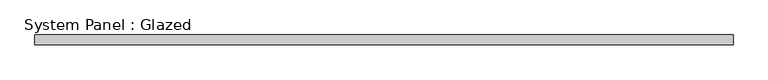
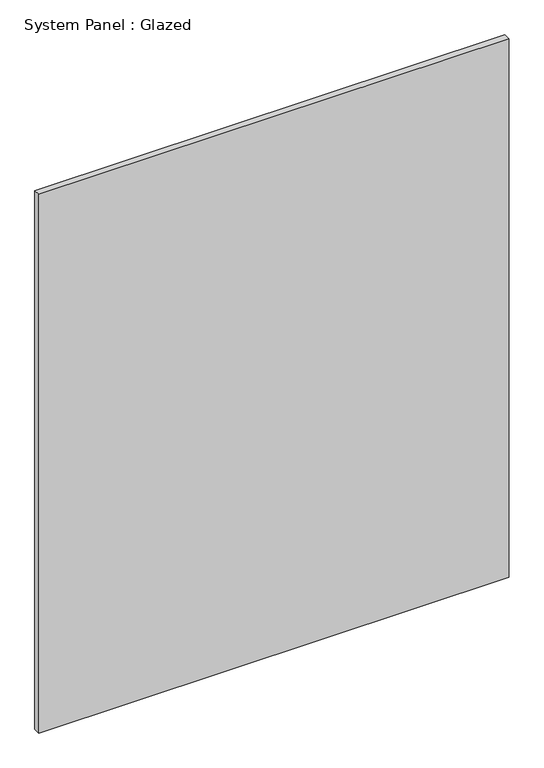
"""IFC4 building model written with IfcOpenShell, lengths in millimetres: plate geometry, System Panel : Glazed."""

from ifc_helpers import new_model, si_unit, origin, origin_with_axes, place, context, project, spatial, polyline, outline, extrude, source, transform, mapped, element, save


def system_panel_glazed_53184239(model_context):
    return source(origin(), model_context, "Body", "SweptSolid", [
        extrude(outline(polyline([(887.9485033, -49.5), (-887.9485033, -49.5), (-887.9485033, -24.5), (887.9485033, -24.5), (887.9485033, -49.5)])), origin_with_axes(), (0.0, 0.0, 1.0), 2150.0),
    ])


if __name__ == "__main__":
    model = new_model("IFC4")
    model_context = context("Model", 3, world=origin())
    ifc_project = project(units=[si_unit("LENGTHUNIT", "METRE", prefix="MILLI")], contexts=[model_context])
    site = spatial("IfcSite", under=ifc_project)
    building = spatial("IfcBuilding", under=site)
    placement = place(None, origin())
    system_panel_glazed_shape = system_panel_glazed_53184239(model_context)
    element("IfcPlate", 1, ObjectType="System Panel : Glazed", at=placement, inside=building, context=model_context, shape_type="MappedRepresentation", body=[
        mapped(system_panel_glazed_shape, transform((0.0, 0.0, 0.0), x_axis=(1.0, 0.0, 0.0), y_axis=(0.0, 1.0, 0.0), z_axis=(0.0, 0.0, 1.0))),
    ])
    save(model, "model.ifc")

# Revit data of these elements
# Type "System Panel : Glazed"
#   Keynote = "H11"
#   Construction Type Id = "GSP4R"
#   Analytic Construction = "1/8 in Pilkington single glazing"
#   Visual Light Transmittance = 0.9
#   Solar Heat Gain Coefficient = 0.86
#   Heat Transfer Coefficient (U) = 6.7069 W/(m²·K)
# Element 1 (IfcPlate, "System Panel : Glazed")
#   Materials on its faces: "Glass"
# Materials
#   "Glass": class "Glass", colour RGB 0 128 192, transparency 0.9, Description = "Soda Lime Glass", Cost = 0
